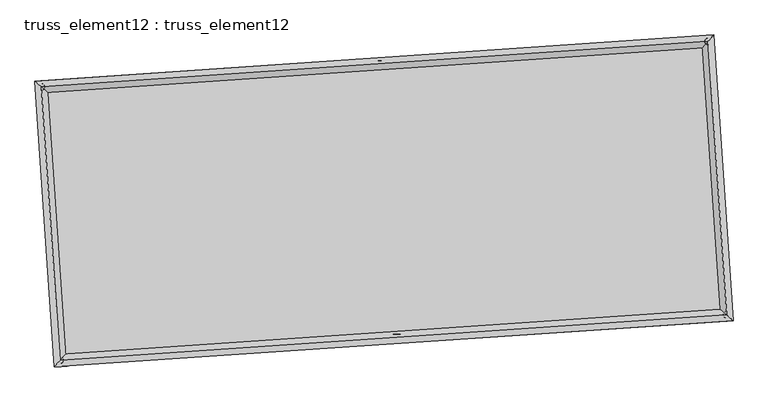
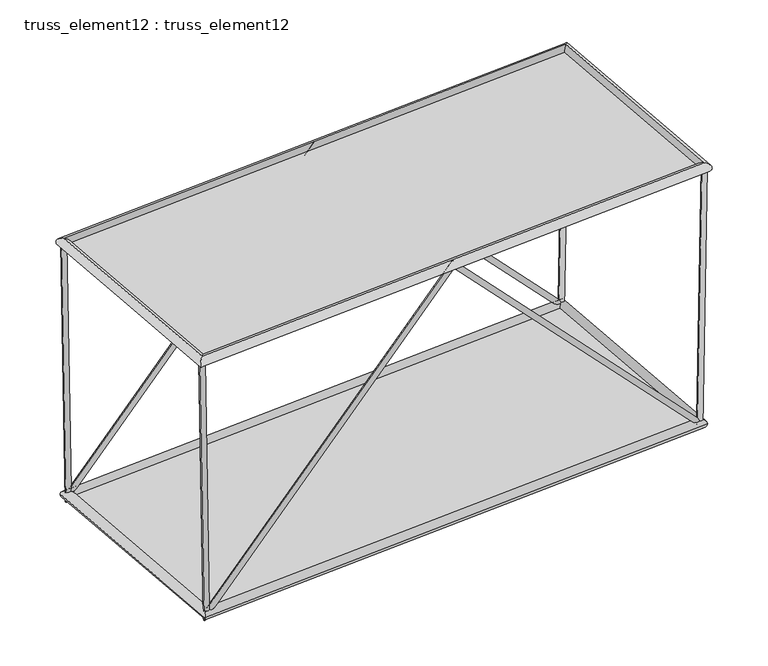
"""IFC4 building model written with IfcOpenShell, lengths in millimetres: plate geometry, truss_element12 : truss_element12."""

from ifc_helpers import new_model, si_unit, frame, origin, origin_with_axes, place, context, project, spatial, polyline, circle_curve, ellipse_curve, outline, extrude, source, transform, mapped, element, save
from ifc_brep_helpers import plane_surface, cylinder_surface, advanced_brep


def truss_element12_truss_element12_d2dc27e5(model_context):
    return source(origin(), model_context, "Body", "SolidModel", [
        advanced_brep(
        [(-3750.4936923, 2270.3904911, 5000.120325), (-3849.582422, 2257.0302647, 4998.409186), (-3667.0221146, 2276.0821006, 122.0048198), (-3761.9647682, 2263.0045795, -122.0048198), (1064.434046, 2598.7021103, 5071.3707956), (1064.871576, 2592.1282012, 4927.1341263), (5794.4951758, 2921.2269981, 121.9949961), (5890.2658012, 2921.1534904, -121.9949961), (5879.3513588, 2927.0130186, 5000.1099238), (5979.3359995, 2927.2268486, 4998.3704092)],
        [
            (0, 1, circle_curve(frame((-3800.0380572, 2263.7103779, 4999.2647555), z_axis=(-0.01710892315204124, -0.0011665924326349144, 0.9998529510936465), x_axis=(-0.13360257959464636, 0.9910343456266016, -0.00112982923926399)), 50.0)),
            (1, 0, circle_curve(frame((-3800.0380572, 2263.7103779, 4999.2647555), z_axis=(-0.01710892315204124, -0.0011665924326349144, 0.9998529510936465), x_axis=(-0.13360257959464636, 0.9910343456266016, -0.00112982923926399)), 50.0)),
            (0, 2),
            (2, 3, ellipse_curve(frame((-3714.4934414, 2269.54334, 0.0), z_axis=(-0.9289170101606278, -0.06333931977871671, 0.3648305343638462), x_axis=(0.36398536651593416, 0.024818778504806103, 0.9310739397039263)), 131.3219892, 50.0)),
            (3, 1),
            (3, 2, ellipse_curve(frame((-3714.4934414, 2269.54334, 0.0), z_axis=(-0.9289170101606278, -0.06333931977871671, 0.3648305343638462), x_axis=(0.36398536651593416, 0.024818778504806103, 0.9310739397039263)), 131.3219892, 50.0)),
            (2, 4),
            (4, 5, ellipse_curve(frame((1064.652811, 2595.4151558, 4999.252461), z_axis=(-0.9976833933321771, -0.06802823804168875, 7.414941499714515e-05), x_axis=(-7.39776401714257e-05, -5.0442540650833885e-06, -0.9999999972509322)), 72.2753704, 50.0)),
            (5, 3),
            (5, 4, ellipse_curve(frame((1064.652811, 2595.4151558, 4999.252461), z_axis=(-0.9976833933321771, -0.06802823804168875, 7.414941499714515e-05), x_axis=(-7.39776401714257e-05, -5.0442540650833885e-06, -0.9999999972509322)), 72.2753704, 50.0)),
            (4, 6),
            (6, 7, ellipse_curve(frame((5842.3804885, 2921.1902443, 0.0), z_axis=(-0.9289957394028395, -0.06334468802646322, -0.3646290809441854), x_axis=(-0.36378437978405576, -0.02480507398358674, 0.931152851754103)), 131.300287, 50.0)),
            (7, 5),
            (7, 6, ellipse_curve(frame((5842.3804885, 2921.1902443, 0.0), z_axis=(-0.9289957394028395, -0.06334468802646322, -0.3646290809441854), x_axis=(-0.36378437978405576, -0.02480507398358674, 0.931152851754103)), 131.300287, 50.0)),
            (8, 9, circle_curve(frame((5929.3436792, 2927.1199336, 4999.2401665), z_axis=(0.017392638132466113, 0.001185937878642774, 0.9998480332981313), x_axis=(-0.002158604726762429, 0.9999970106075159, -0.0011485650461673309)), 50.0)),
            (9, 8, circle_curve(frame((5929.3436792, 2927.1199336, 4999.2401665), z_axis=(0.017392638132466113, 0.001185937878642774, 0.9998480332981313), x_axis=(-0.002158604726762429, 0.9999970106075159, -0.0011485650461673309)), 50.0)),
            (6, 8),
            (9, 7),
        ],
        [
            plane_surface(frame((-3800.0380572, 2313.7103439, 4999.3230936), z_axis=(-0.01710892315204017, -0.001166592432634736, 0.9998529510936465), x_axis=(0.9998536316624437, -1.9962062093981113e-05, 0.017108911506536383))),
            cylinder_surface(frame((-3800.0380572, 2263.7103779, 4999.2647555), z_axis=(-0.017108923152041242, -0.0011665924326349146, 0.9998529510936467), x_axis=(-0.13360257959464636, 0.9910343456266016, -0.00112982923926399)), 50.0),
            cylinder_surface(frame((-3714.4934414, 2269.54334, 0.0), z_axis=(-0.69024939212398, -0.04706548216534755, -0.7220392074264527), x_axis=(-0.020419483033555893, 0.998751870731873, -0.045582292858373695)), 50.0),
            cylinder_surface(frame((1064.652811, 2595.4151558, 4999.252461), z_axis=(-0.6901425550207504, -0.04705819734940832, 0.7221418003492492), x_axis=(-0.11534812165123533, 0.9922790477220719, -0.045575237611120895)), 50.0),
            plane_surface(frame((5929.3436792, 2877.1199688, 4999.2994724), z_axis=(0.01739263813246562, 0.001185937878642426, 0.9998480332981314), x_axis=(0.9998487366290929, -2.0629708890496073e-05, -0.017392625897834066))),
            cylinder_surface(frame((5842.3804885, 2921.1902443, 0.0), z_axis=(-0.017392638132466113, -0.001185937878642774, -0.9998480332981313), x_axis=(-0.002158604726762429, 0.9999970106075159, -0.0011485650461673309)), 50.0),
        ],
        [
            (0, [[1, 2]]),
            (1, [[-1, 3, 4, 5]]),
            (1, [[-2, -5, 6, -3]]),
            (2, [[-4, 7, 8, 9]]),
            (2, [[-6, -9, 10, -7]]),
            (3, [[-8, 11, 12, 13]]),
            (3, [[-10, -13, 14, -11]]),
            (4, [[15, 16]]),
            (5, [[-12, 17, -16, 18]]),
            (5, [[-14, -18, -15, -17]]),
        ],
    ),
        advanced_brep(
        [(-3478.3807394, -1720.3430932, 5000.120325), (-3577.4694691, -1733.7033196, 4998.409186), (-3394.9091617, -1714.6514837, 122.0048198), (-3489.8518153, -1727.7290048, -122.0048198), (1336.5469989, -1392.031474, 5071.3707956), (1336.9845289, -1398.6053831, 4927.1341263), (6066.6081287, -1069.5065862, 121.9949961), (6162.3787541, -1069.5800939, -121.9949961), (6151.4643118, -1063.7205657, 5000.1099238), (6251.4489524, -1063.5067356, 4998.3704092)],
        [
            (0, 1, circle_curve(frame((-3527.9251043, -1727.0232064, 4999.2647555), z_axis=(-0.017108923152041454, -0.0011665924326349345, 0.9998529510936464), x_axis=(-0.1336025795946458, 0.9910343456266016, -0.0011298292392639894)), 50.0)),
            (1, 0, circle_curve(frame((-3527.9251043, -1727.0232064, 4999.2647555), z_axis=(-0.017108923152041454, -0.0011665924326349345, 0.9998529510936464), x_axis=(-0.1336025795946458, 0.9910343456266016, -0.0011298292392639894)), 50.0)),
            (0, 2),
            (2, 3, ellipse_curve(frame((-3442.3804885, -1721.1902443, 0.0), z_axis=(-0.9289170101606279, -0.06333931977871649, 0.36483053436384594), x_axis=(0.36398536651593394, 0.024818778504805978, 0.9310739397039264)), 131.3219892, 50.0)),
            (3, 1),
            (3, 2, ellipse_curve(frame((-3442.3804885, -1721.1902443, 0.0), z_axis=(-0.9289170101606279, -0.06333931977871649, 0.36483053436384594), x_axis=(0.36398536651593394, 0.024818778504805978, 0.9310739397039264)), 131.3219892, 50.0)),
            (2, 4),
            (4, 5, ellipse_curve(frame((1336.7657639, -1395.3184285, 4999.252461), z_axis=(-0.9976833933321771, -0.0680282380416885, 7.414941499714518e-05), x_axis=(-7.397764017142569e-05, -5.0442540650641685e-06, -0.9999999972509322)), 72.2753704, 50.0)),
            (5, 3),
            (5, 4, ellipse_curve(frame((1336.7657639, -1395.3184285, 4999.252461), z_axis=(-0.9976833933321771, -0.0680282380416885, 7.414941499714518e-05), x_axis=(-7.397764017142569e-05, -5.0442540650641685e-06, -0.9999999972509322)), 72.2753704, 50.0)),
            (4, 6),
            (6, 7, ellipse_curve(frame((6114.4934414, -1069.54334, 0.0), z_axis=(-0.9289957394028399, -0.06334468802646308, -0.3646290809441853), x_axis=(-0.36378437978405553, -0.02480507398358664, 0.9311528517541031)), 131.300287, 50.0)),
            (7, 5),
            (7, 6, ellipse_curve(frame((6114.4934414, -1069.54334, 0.0), z_axis=(-0.9289957394028399, -0.06334468802646308, -0.3646290809441853), x_axis=(-0.36378437978405553, -0.02480507398358664, 0.9311528517541031)), 131.300287, 50.0)),
            (8, 9, circle_curve(frame((6201.4566321, -1063.6136507, 4999.2401665), z_axis=(0.01739263813246659, 0.0011859378786428217, 0.9998480332981314), x_axis=(-0.00215860472676268, 0.999997010607516, -0.0011485650461673731)), 50.0)),
            (9, 8, circle_curve(frame((6201.4566321, -1063.6136507, 4999.2401665), z_axis=(0.01739263813246659, 0.0011859378786428217, 0.9998480332981314), x_axis=(-0.00215860472676268, 0.999997010607516, -0.0011485650461673731)), 50.0)),
            (6, 8),
            (9, 7),
        ],
        [
            plane_surface(frame((-3527.9251043, -1677.0232404, 4999.3230936), z_axis=(-0.01710892315204017, -0.0011665924326347264, 0.9998529510936465), x_axis=(0.9998536316624437, -1.9962062093981113e-05, 0.017108911506536383))),
            cylinder_surface(frame((-3527.9251043, -1727.0232064, 4999.2647555), z_axis=(-0.017108923152041457, -0.0011665924326349348, 0.9998529510936466), x_axis=(-0.1336025795946458, 0.9910343456266016, -0.0011298292392639894)), 50.0),
            cylinder_surface(frame((-3442.3804885, -1721.1902443, 0.0), z_axis=(-0.6902493921239796, -0.04706548216534734, -0.7220392074264529), x_axis=(-0.02041948303355586, 0.998751870731873, -0.04558229285837343)), 50.0),
            cylinder_surface(frame((1336.7657639, -1395.3184285, 4999.252461), z_axis=(-0.6901425550207501, -0.04705819734940815, 0.7221418003492494), x_axis=(-0.11534812165123483, 0.9922790477220719, -0.04557523761112062)), 50.0),
            plane_surface(frame((6201.4566321, -1113.6136155, 4999.2994724), z_axis=(0.01739263813246562, 0.0011859378786424177, 0.9998480332981314), x_axis=(0.9998487366290929, -2.0629708890051984e-05, -0.017392625897834066))),
            cylinder_surface(frame((6114.4934414, -1069.54334, 0.0), z_axis=(-0.01739263813246659, -0.0011859378786428217, -0.9998480332981314), x_axis=(-0.00215860472676268, 0.999997010607516, -0.0011485650461673731)), 50.0),
        ],
        [
            (0, [[1, 2]]),
            (1, [[-1, 3, 4, 5]]),
            (1, [[-2, -5, 6, -3]]),
            (2, [[-4, 7, 8, 9]]),
            (2, [[-6, -9, 10, -7]]),
            (3, [[-8, 11, 12, 13]]),
            (3, [[-10, -13, 14, -11]]),
            (4, [[15, 16]]),
            (5, [[-12, 17, -16, 18]]),
            (5, [[-14, -18, -15, -17]]),
        ],
    ),
        advanced_brep(
        [(-3527.9315258, -1727.0303236, 4909.2647557), (-3527.9186827, -1727.0160892, 5089.2647552), (-3800.030729, 2263.7041982, 5089.2647552), (-3800.0453854, 2263.7165576, 4909.2647557), (5929.3377104, 2927.1128473, 5089.2401663), (5929.3496479, 2927.12702, 4909.2401667), (6201.4497567, -1063.6074401, 5089.2401663), (6201.4635075, -1063.6198612, 4909.2401667)],
        [
            (0, 1, ellipse_curve(frame((-3527.9251043, -1727.0232064, 4999.2647555), z_axis=(-0.7535719234032141, 0.6573654662782353, 1.7829245935204696e-06), x_axis=(-0.6573654662758399, -0.7535719234053034, 1.7829245812694147e-06)), 127.2792206, 90.0)),
            (1, 2),
            (2, 3, ellipse_curve(frame((-3800.0380572, 2263.7103779, 4999.2647555), z_axis=(-0.6573654662758396, -0.753571923405304, 1.7829245811910703e-06), x_axis=(0.7535719234032143, -0.6573654662782349, -1.7829245934421267e-06)), 127.2792206, 90.0)),
            (3, 0),
            (1, 0, ellipse_curve(frame((-3527.9251043, -1727.0232064, 4999.2647555), z_axis=(-0.7535719234032141, 0.6573654662782353, 1.7829245935204696e-06), x_axis=(-0.6573654662758399, -0.7535719234053034, 1.7829245812694147e-06)), 127.2792206, 90.0)),
            (3, 2, ellipse_curve(frame((-3800.0380572, 2263.7103779, 4999.2647555), z_axis=(-0.6573654662758396, -0.753571923405304, 1.7829245811910703e-06), x_axis=(0.7535719234032143, -0.6573654662782349, -1.7829245934421267e-06)), 127.2792206, 90.0)),
            (2, 4),
            (4, 5, ellipse_curve(frame((5929.3436792, 2927.1199336, 4999.2401665), z_axis=(-0.7535719234032134, 0.6573654662782358, 1.782924593633729e-06), x_axis=(-0.6573654662758406, -0.753571923405303, 1.7829245809994683e-06)), 127.2792206, 90.0)),
            (5, 3),
            (5, 4, ellipse_curve(frame((5929.3436792, 2927.1199336, 4999.2401665), z_axis=(-0.7535719234032134, 0.6573654662782358, 1.782924593633729e-06), x_axis=(-0.6573654662758406, -0.753571923405303, 1.7829245809994683e-06)), 127.2792206, 90.0)),
            (4, 6),
            (6, 7, ellipse_curve(frame((6201.4566321, -1063.6136507, 4999.2401665), z_axis=(0.6573654662758406, 0.7535719234053031, -1.7829245810778119e-06), x_axis=(-0.7535719234032136, 0.6573654662782359, 1.7829245937120725e-06)), 127.2792206, 90.0)),
            (7, 5),
            (7, 6, ellipse_curve(frame((6201.4566321, -1063.6136507, 4999.2401665), z_axis=(0.6573654662758406, 0.7535719234053031, -1.7829245810778119e-06), x_axis=(-0.7535719234032136, 0.6573654662782359, 1.7829245937120725e-06)), 127.2792206, 90.0)),
            (6, 1),
            (0, 7),
        ],
        [
            cylinder_surface(frame((-3527.9251043, -1727.0232064, 4999.2647555), z_axis=(0.06802823822869955, -0.9976833960748767, 0.0), x_axis=(-0.9976833931505921, -0.0680282380293037, 7.65646749386812e-05)), 90.0),
            cylinder_surface(frame((-3800.0380572, 2263.7103779, 4999.2647555), z_axis=(-0.9976833960717053, -0.06802823822848321, 2.5214361320715873e-06), x_axis=(-0.06802823785595762, 0.9976833933527269, 7.404323882218444e-05)), 90.0),
            cylinder_surface(frame((5929.3436792, 2927.1199336, 4999.2401665), z_axis=(-0.06802823822869739, 0.997683396074877, 0.0), x_axis=(0.997683393523118, 0.06802823805470264, 7.152180268809107e-05)), 90.0),
            cylinder_surface(frame((6201.4566321, -1063.6136507, 4999.2401665), z_axis=(0.9976833960717054, 0.06802823822848272, -2.5214361321823818e-06), x_axis=(0.06802823822848272, -0.9976833933273259, 7.404323880442816e-05)), 90.0),
        ],
        [
            (0, [[1, 2, 3, 4]]),
            (0, [[5, -4, 6, -2]]),
            (1, [[-3, 7, 8, 9]]),
            (1, [[-6, -9, 10, -7]]),
            (2, [[-8, 11, 12, 13]]),
            (2, [[-10, -13, 14, -11]]),
            (3, [[-12, 15, -1, 16]]),
            (3, [[-14, -16, -5, -15]]),
        ],
    ),
        advanced_brep(
        [(-3358.7115243, -1625.2761972, 0.0), (-3526.0494527, -1817.1042913, 0.0), (-3810.4074885, 2353.2123043, 0.0), (-3618.5793943, 2185.8743758, 0.0), (5926.0494527, 3017.1042913, 0.0), (5758.7115243, 2825.2761972, 0.0), (6210.4074885, -1153.2123043, 0.0), (6018.5793943, -985.8743758, 0.0)],
        [
            (0, 1, ellipse_curve(frame((-3442.3804885, -1721.1902443, 0.0), z_axis=(-0.7535719234054589, 0.6573654662780798, 0.0), x_axis=(-0.6573654662780798, -0.7535719234054589, 0.0)), 127.2792206, 90.0)),
            (1, 2),
            (2, 3, ellipse_curve(frame((-3714.4934414, 2269.54334, 0.0), z_axis=(-0.6573654662780795, -0.753571923405459, 0.0), x_axis=(0.7535719234054589, -0.6573654662780798, 0.0)), 127.2792206, 90.0)),
            (3, 0),
            (1, 0, ellipse_curve(frame((-3442.3804885, -1721.1902443, 0.0), z_axis=(-0.7535719234054589, 0.6573654662780798, 0.0), x_axis=(-0.6573654662780798, -0.7535719234054589, 0.0)), 127.2792206, 90.0)),
            (3, 2, ellipse_curve(frame((-3714.4934414, 2269.54334, 0.0), z_axis=(-0.6573654662780795, -0.753571923405459, 0.0), x_axis=(0.7535719234054589, -0.6573654662780798, 0.0)), 127.2792206, 90.0)),
            (2, 4),
            (4, 5, ellipse_curve(frame((5842.3804885, 2921.1902443, 0.0), z_axis=(-0.7535719234054582, 0.6573654662780805, 0.0), x_axis=(-0.6573654662780805, -0.7535719234054581, 0.0)), 127.2792206, 90.0)),
            (5, 3),
            (5, 4, ellipse_curve(frame((5842.3804885, 2921.1902443, 0.0), z_axis=(-0.7535719234054582, 0.6573654662780805, 0.0), x_axis=(-0.6573654662780805, -0.7535719234054581, 0.0)), 127.2792206, 90.0)),
            (4, 6),
            (6, 7, ellipse_curve(frame((6114.4934414, -1069.54334, 0.0), z_axis=(0.6573654662780807, 0.7535719234054581, 0.0), x_axis=(-0.7535719234054581, 0.6573654662780806, 0.0)), 127.2792206, 90.0)),
            (7, 5),
            (7, 6, ellipse_curve(frame((6114.4934414, -1069.54334, 0.0), z_axis=(0.6573654662780807, 0.7535719234054581, 0.0), x_axis=(-0.7535719234054581, 0.6573654662780806, 0.0)), 127.2792206, 90.0)),
            (6, 1),
            (0, 7),
        ],
        [
            cylinder_surface(frame((-3442.3804885, -1721.1902443, 0.0), z_axis=(0.06802823822870281, -0.9976833960748764, 0.0), x_axis=(-0.9976833960748764, -0.06802823822870281, 0.0)), 90.0),
            cylinder_surface(frame((-3714.4934414, 2269.54334, 0.0), z_axis=(-0.9976833960748764, -0.06802823822870283, 0.0), x_axis=(-0.06802823822870283, 0.9976833960748764, 0.0)), 90.0),
            cylinder_surface(frame((5842.3804885, 2921.1902443, 0.0), z_axis=(-0.06802823822870042, 0.9976833960748767, 0.0), x_axis=(0.9976833960748767, 0.06802823822870042, 0.0)), 90.0),
            cylinder_surface(frame((6114.4934414, -1069.54334, 0.0), z_axis=(0.9976833960748765, 0.06802823822870231, 0.0), x_axis=(0.06802823822870231, -0.9976833960748765, 0.0)), 90.0),
        ],
        [
            (0, [[1, 2, 3, 4]]),
            (0, [[5, -4, 6, -2]]),
            (1, [[-3, 7, 8, 9]]),
            (1, [[-6, -9, 10, -7]]),
            (2, [[-8, 11, 12, 13]]),
            (2, [[-10, -13, 14, -11]]),
            (3, [[-12, 15, -1, 16]]),
            (3, [[-14, -16, -5, -15]]),
        ],
    ),
        extrude(outline(polyline([(-3442.3804885, -1721.1902443), (-3714.4934414, 2269.54334), (5842.3804885, 2921.1902443), (6114.4934414, -1069.54334), (-3442.3804885, -1721.1902443)])), origin_with_axes(), (0.0, 0.0, 1.0), 20.0),
        extrude(outline(polyline([(-2000.0, 4875.986598), (2000.0, 4875.9865979), (2000.0, -4875.9865979), (-2000.0, -4875.9865978), (-2000.0, 4875.986598)])), frame((1200.7092875, 600.0483636, 4999.252461), z_axis=(2.515594963820283e-06, 1.7152884922814844e-07, 0.9999999999968212), x_axis=(-0.06802823822870298, 0.9976833960748764, 0.0)), (0.0, 0.0, 1.0), 20.0),
    ])


if __name__ == "__main__":
    model = new_model("IFC4")
    model_context = context("Model", 3, world=origin())
    ifc_project = project(units=[si_unit("LENGTHUNIT", "METRE", prefix="MILLI")], contexts=[model_context])
    site = spatial("IfcSite", under=ifc_project)
    building = spatial("IfcBuilding", under=site)
    placement = place(None, origin())
    truss_element12_truss_element12_shape = truss_element12_truss_element12_d2dc27e5(model_context)
    element("IfcPlate", 1, ObjectType="truss_element12 : truss_element12", at=placement, inside=building, context=model_context, shape_type="MappedRepresentation", body=[
        mapped(truss_element12_truss_element12_shape, transform((0.0, 0.0, 0.0), x_axis=(1.0, 0.0, 0.0), y_axis=(0.0, 1.0, 0.0), z_axis=(0.0, 0.0, 1.0))),
    ])
    save(model, "model.ifc")

# Revit data of these elements
# Type "truss_element12 : truss_element12"
#   steellbar1 = 90 mm
#   steelbar2 = 50 mm
#   offset1 = 5000 mm
#   M = Default Roof
# Element 1 (IfcPlate, "truss_element12 : truss_element12")
#   Materials on its faces: "Default Roof"
# Materials
#   "Default Roof": class "Miscellaneous", colour RGB 0 127 0, transparency 0, Comments = "Rendering appearance not upgraded Rendering appearance not upgraded ", Cost = 0
